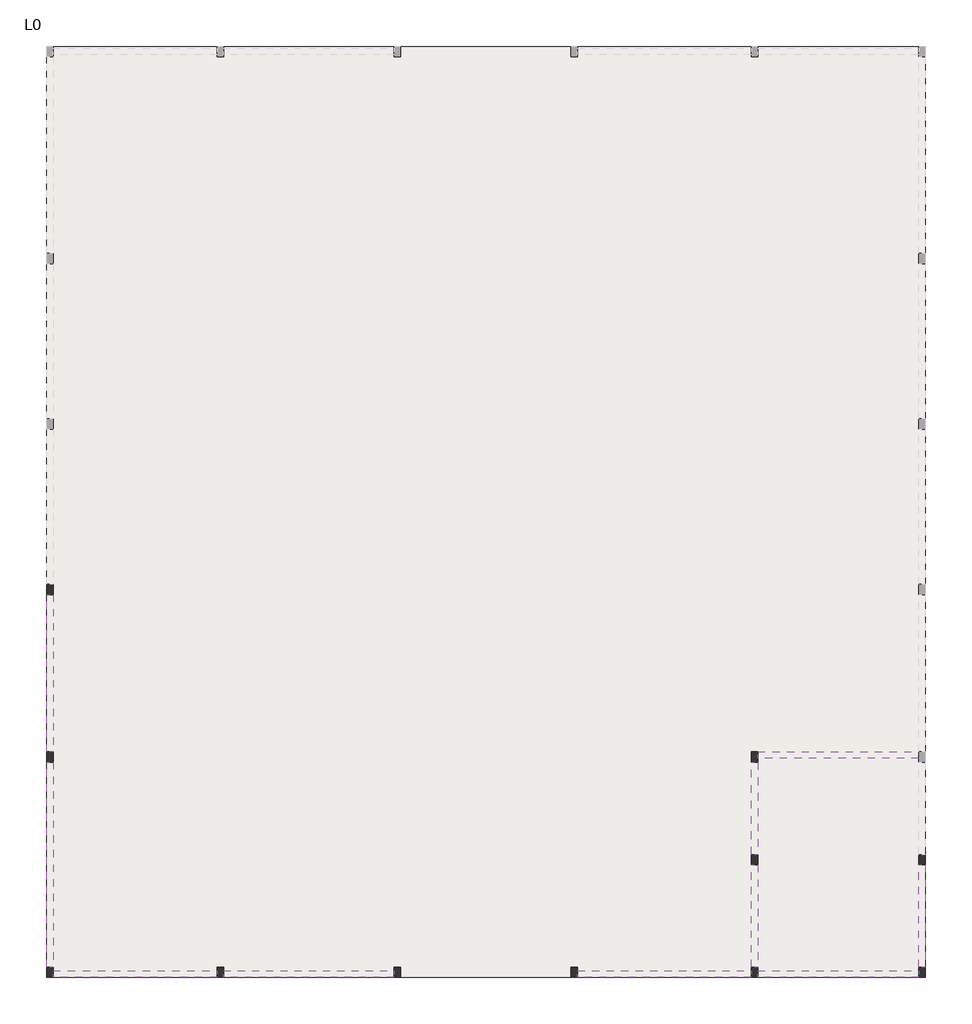
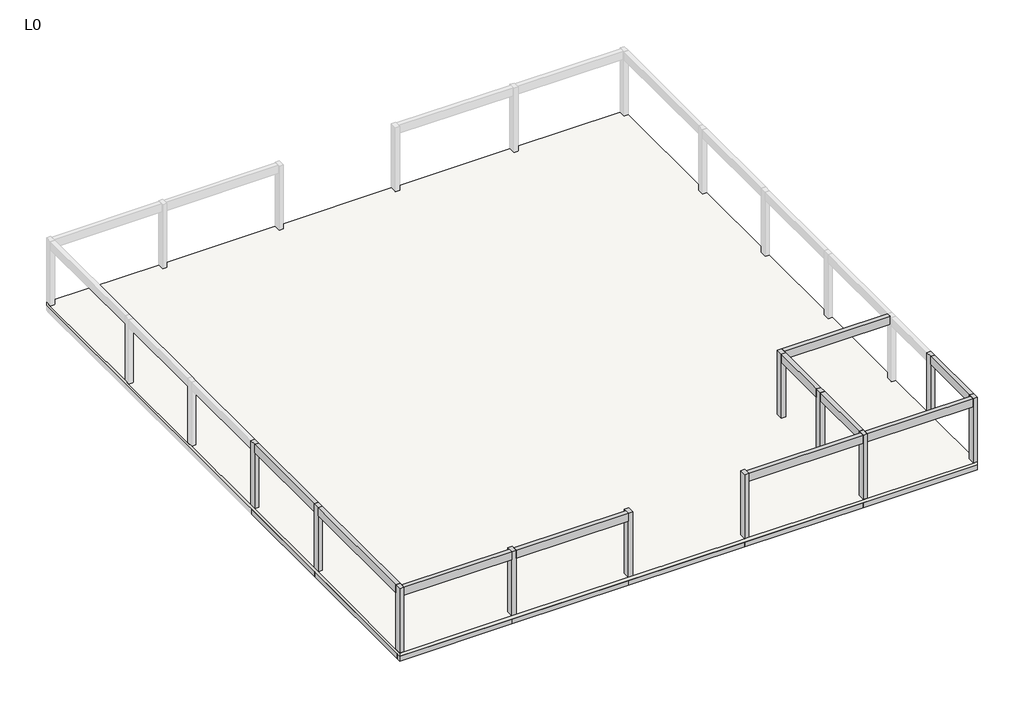
# One storey, part 1 of 2: 32 beams, 11 columns, 1 slab.
"""IFC4 building model written with IfcOpenShell, lengths in millimetres."""

from ifc_helpers import new_model, si_unit, frame, origin, origin_with_axes, place, context, project, spatial, polyline, outline, extrude, faceted_brep, element, save

model = new_model("IFC4")

# Units and contexts
model_context = context("Model", 3, world=origin())
ifc_project = project(units=[si_unit("LENGTHUNIT", "METRE", prefix="MILLI")], contexts=[model_context])

# Site, building, storey
site = spatial("IfcSite", under=ifc_project)
building = spatial("IfcBuilding", under=site)
storey = spatial("IfcBuildingStorey", under=building, Name="L0", Elevation=0.0)

# Beams
placement = place(None, origin())
element("IfcBeam", 1, ObjectType="Concrete-Rectangular Beam : 25 x 50", at=placement, inside=storey, context=model_context, shape_type="Brep", body=[
    faceted_brep([(17000.0, -2875.0, -500.0), (16750.0, -2875.0, -500.0), (10520.0, -2875.0, -500.0), (10520.0, -2875.0, -200.0), (16750.0, -2875.0, -200.0), (17000.0, -2875.0, -200.0), (17000.0, -3125.0, -500.0), (16750.0, -3125.0, -500.0), (10520.0, -3125.0, -500.0), (17000.0, -3125.0, -200.0), (16750.0, -3125.0, -200.0), (10520.0, -3125.0, -200.0)], [[[0, 1, 2, 3, 4, 5]], [[0, 6, 7, 8, 2, 1]], [[8, 7, 6, 9, 10, 11]], [[6, 0, 5, 9]], [[2, 8, 11, 3]], [[5, 4, 3, 11, 10, 9]]]),
])
element("IfcBeam", 2, ObjectType="Concrete-Rectangular Beam : 25 x 50", at=placement, inside=storey, context=model_context, shape_type="Brep", body=[
    faceted_brep([(17000.0, -9345.0, -500.0), (16750.0, -9345.0, -500.0), (10520.0, -9345.0, -500.0), (10270.0, -9345.0, -500.0), (10270.0, -9345.0, -200.0), (10520.0, -9345.0, -200.0), (16750.0, -9345.0, -200.0), (17000.0, -9345.0, -200.0), (10270.0, -9595.0, -500.0), (17000.0, -9595.0, -500.0), (16750.0, -9595.0, -500.0), (10520.0, -9595.0, -500.0), (17000.0, -9595.0, -200.0), (16750.0, -9595.0, -200.0), (10520.0, -9595.0, -200.0), (10270.0, -9595.0, -200.0)], [[[0, 1, 2, 3, 4, 5, 6, 7]], [[8, 3, 2, 1, 0, 9, 10, 11]], [[8, 11, 10, 9, 12, 13, 14, 15]], [[3, 8, 15, 4]], [[9, 0, 7, 12]], [[7, 6, 5, 4, 15, 14, 13, 12]]]),
])
element("IfcBeam", 3, ObjectType="Concrete-Rectangular Beam : 25 x 50", at=placement, inside=storey, context=model_context, shape_type="Brep", body=[
    faceted_brep([(10270.0, -9345.0, -500.0), (3550.0, -9345.0, -500.0), (3300.0, -9345.0, -500.0), (-3300.0, -9345.0, -500.0), (-3300.0, -9345.0, -200.0), (3300.0, -9345.0, -200.0), (3550.0, -9345.0, -200.0), (10270.0, -9345.0, -200.0), (10270.0, -9595.0, -500.0), (3550.0, -9595.0, -500.0), (3300.0, -9595.0, -500.0), (-3300.0, -9595.0, -500.0), (10270.0, -9595.0, -200.0), (3550.0, -9595.0, -200.0), (3300.0, -9595.0, -200.0), (-3300.0, -9595.0, -200.0)], [[[0, 1, 2, 3, 4, 5, 6, 7]], [[0, 8, 9, 10, 11, 3, 2, 1]], [[11, 10, 9, 8, 12, 13, 14, 15]], [[8, 0, 7, 12]], [[3, 11, 15, 4]], [[7, 6, 5, 4, 15, 14, 13, 12]]]),
])
element("IfcBeam", 4, ObjectType="Concrete-Rectangular Beam : 25 x 50", at=placement, inside=storey, context=model_context, shape_type="Brep", body=[
    faceted_brep([(17000.0, -17750.0, -500.0), (16750.0, -17750.0, -500.0), (10520.0, -17750.0, -500.0), (10270.0, -17750.0, -500.0), (10270.0, -17750.0, -200.0), (10520.0, -17750.0, -200.0), (16750.0, -17750.0, -200.0), (17000.0, -17750.0, -200.0), (10270.0, -18000.0, -500.0), (17000.0, -18000.0, -500.0), (17000.0, -18000.0, -200.0), (10270.0, -18000.0, -200.0)], [[[0, 1, 2, 3, 4, 5, 6, 7]], [[8, 3, 2, 1, 0, 9]], [[8, 9, 10, 11]], [[3, 8, 11, 4]], [[9, 0, 7, 10]], [[7, 6, 5, 4, 11, 10]]]),
])
element("IfcBeam", 5, ObjectType="Concrete-Rectangular Beam : 25 x 50", at=placement, inside=storey, context=model_context, shape_type="Brep", body=[
    faceted_brep([(10270.0, -17750.0, -500.0), (3550.0, -17750.0, -500.0), (3300.0, -17750.0, -500.0), (3300.0, -17750.0, -200.0), (3550.0, -17750.0, -200.0), (10270.0, -17750.0, -200.0), (3300.0, -18000.0, -500.0), (10270.0, -18000.0, -500.0), (10270.0, -18000.0, -200.0), (3300.0, -18000.0, -200.0)], [[[0, 1, 2, 3, 4, 5]], [[6, 2, 1, 0, 7]], [[6, 7, 8, 9]], [[2, 6, 9, 3]], [[7, 0, 5, 8]], [[5, 4, 3, 9, 8]]]),
])
element("IfcBeam", 6, ObjectType="Concrete-Rectangular Beam : 25 x 50", at=placement, inside=storey, context=model_context, shape_type="Brep", body=[
    faceted_brep([(3300.0, -17750.0, -500.0), (-3300.0, -17750.0, -500.0), (-3550.0, -17750.0, -500.0), (-3550.0, -17750.0, -200.0), (-3300.0, -17750.0, -200.0), (3300.0, -17750.0, -200.0), (-3550.0, -18000.0, -500.0), (3300.0, -18000.0, -500.0), (3300.0, -18000.0, -200.0), (-3550.0, -18000.0, -200.0)], [[[0, 1, 2, 3, 4, 5]], [[6, 2, 1, 0, 7]], [[6, 7, 8, 9]], [[2, 6, 9, 3]], [[7, 0, 5, 8]], [[5, 4, 3, 9, 8]]]),
])
element("IfcBeam", 7, ObjectType="Concrete-Rectangular Beam : 25 x 50", at=placement, inside=storey, context=model_context, shape_type="Brep", body=[
    faceted_brep([(-3550.0, -17750.0, -500.0), (-10150.0, -17750.0, -500.0), (-10400.0, -17750.0, -500.0), (-10400.0, -17750.0, -200.0), (-10150.0, -17750.0, -200.0), (-3550.0, -17750.0, -200.0), (-10400.0, -18000.0, -500.0), (-3550.0, -18000.0, -500.0), (-3550.0, -18000.0, -200.0), (-10400.0, -18000.0, -200.0)], [[[0, 1, 2, 3, 4, 5]], [[6, 2, 1, 0, 7]], [[6, 7, 8, 9]], [[2, 6, 9, 3]], [[7, 0, 5, 8]], [[5, 4, 3, 9, 8]]]),
])
element("IfcBeam", 8, ObjectType="Concrete-Rectangular Beam : 25 x 50", at=placement, inside=storey, context=model_context, shape_type="Brep", body=[
    faceted_brep([(-10400.0, -17750.0, -500.0), (-16750.0, -17750.0, -500.0), (-17000.0, -17750.0, -500.0), (-17000.0, -17750.0, -200.0), (-16750.0, -17750.0, -200.0), (-10400.0, -17750.0, -200.0), (-10400.0, -18000.0, -500.0), (-17000.0, -18000.0, -500.0), (-10400.0, -18000.0, -200.0), (-17000.0, -18000.0, -200.0)], [[[0, 1, 2, 3, 4, 5]], [[0, 6, 7, 2, 1]], [[7, 6, 8, 9]], [[6, 0, 5, 8]], [[2, 7, 9, 3]], [[5, 4, 3, 9, 8]]]),
])
element("IfcBeam", 9, ObjectType="Concrete-Rectangular Beam : 25 x 50", at=placement, inside=storey, context=model_context, shape_type="Brep", body=[
    faceted_brep([(-16750.0, -17750.0, -500.0), (-16750.0, -9595.0, -500.0), (-16750.0, -9345.0, -500.0), (-16750.0, -9345.0, -200.0), (-16750.0, -9595.0, -200.0), (-16750.0, -17750.0, -200.0), (-17000.0, -9345.0, -500.0), (-17000.0, -17750.0, -500.0), (-17000.0, -17750.0, -200.0), (-17000.0, -9345.0, -200.0)], [[[0, 1, 2, 3, 4, 5]], [[6, 2, 1, 0, 7]], [[6, 7, 8, 9]], [[2, 6, 9, 3]], [[7, 0, 5, 8]], [[5, 4, 3, 9, 8]]]),
])
element("IfcBeam", 10, ObjectType="Concrete-Rectangular Beam : 25 x 50", at=placement, inside=storey, context=model_context, shape_type="Brep", body=[
    faceted_brep([(-16750.0, -9345.0, -500.0), (-16750.0, -3125.0, -500.0), (-16750.0, -2875.0, -500.0), (-16750.0, -2875.0, -200.0), (-16750.0, -3125.0, -200.0), (-16750.0, -9345.0, -200.0), (-17000.0, -2875.0, -500.0), (-17000.0, -9345.0, -500.0), (-17000.0, -9345.0, -200.0), (-17000.0, -2875.0, -200.0)], [[[0, 1, 2, 3, 4, 5]], [[6, 2, 1, 0, 7]], [[6, 7, 8, 9]], [[2, 6, 9, 3]], [[7, 0, 5, 8]], [[5, 4, 3, 9, 8]]]),
])
element("IfcBeam", 11, ObjectType="Concrete-Rectangular Beam : 25 x 50", at=placement, inside=storey, context=model_context, shape_type="SweptSolid", body=[
    extrude(outline(polyline([(-10150.0, -17750.0), (-10400.0, -17750.0), (-10400.0, -9595.0), (-10150.0, -9595.0), (-10150.0, -17750.0)])), frame((0.0, 0.0, -500.0), z_axis=(0.0, 0.0, 1.0), x_axis=(1.0, 0.0, 0.0)), (0.0, 0.0, 1.0), 300.0),
])
element("IfcBeam", 12, ObjectType="Concrete-Rectangular Beam : 25 x 50", at=placement, inside=storey, context=model_context, shape_type="Brep", body=[
    faceted_brep([(-3300.0, -17750.0, -500.0), (-3300.0, -9595.0, -500.0), (-3300.0, -9345.0, -500.0), (-3300.0, -3125.0, -500.0), (-3300.0, -2875.0, -500.0), (-3300.0, 3275.0, -500.0), (-3300.0, 3275.0, -200.0), (-3300.0, -2875.0, -200.0), (-3300.0, -3125.0, -200.0), (-3300.0, -9345.0, -200.0), (-3300.0, -9595.0, -200.0), (-3300.0, -17750.0, -200.0), (-3550.0, -17750.0, -500.0), (-3550.0, -9595.0, -500.0), (-3550.0, -9345.0, -500.0), (-3550.0, -3125.0, -500.0), (-3550.0, -2875.0, -500.0), (-3550.0, 3275.0, -500.0), (-3550.0, -17750.0, -200.0), (-3550.0, -9595.0, -200.0), (-3550.0, -9345.0, -200.0), (-3550.0, -3125.0, -200.0), (-3550.0, -2875.0, -200.0), (-3550.0, 3275.0, -200.0)], [[[0, 1, 2, 3, 4, 5, 6, 7, 8, 9, 10, 11]], [[0, 12, 13, 14, 15, 16, 17, 5, 4, 3, 2, 1]], [[17, 16, 15, 14, 13, 12, 18, 19, 20, 21, 22, 23]], [[12, 0, 11, 18]], [[5, 17, 23, 6]], [[11, 10, 9, 8, 7, 6, 23, 22, 21, 20, 19, 18]]]),
])
element("IfcBeam", 13, ObjectType="Concrete-Rectangular Beam : 25 x 50", at=placement, inside=storey, context=model_context, shape_type="SweptSolid", body=[
    extrude(outline(polyline([(3550.0, -17750.0), (3300.0, -17750.0), (3300.0, -9595.0), (3550.0, -9595.0), (3550.0, -17750.0)])), frame((0.0, 0.0, -500.0), z_axis=(0.0, 0.0, 1.0), x_axis=(1.0, 0.0, 0.0)), (0.0, 0.0, 1.0), 300.0),
])
element("IfcBeam", 14, ObjectType="Concrete-Rectangular Beam : 25 x 50", at=placement, inside=storey, context=model_context, shape_type="SweptSolid", body=[
    extrude(outline(polyline([(10270.0, -13448.5675387), (10520.0, -13448.5675387), (10520.0, -17750.0), (10270.0, -17750.0), (10270.0, -13448.5675387)])), frame((0.0, 0.0, -500.0), z_axis=(0.0, 0.0, 1.0), x_axis=(1.0, 0.0, 0.0)), (0.0, 0.0, 1.0), 300.0),
])
element("IfcBeam", 15, ObjectType="Concrete-Rectangular Beam : 25 x 50", at=placement, inside=storey, context=model_context, shape_type="SweptSolid", body=[
    extrude(outline(polyline([(10520.0, -9595.0), (10520.0, -13448.5675387), (10270.0, -13448.5675387), (10270.0, -9595.0), (10520.0, -9595.0)])), frame((0.0, 0.0, -500.0), z_axis=(0.0, 0.0, 1.0), x_axis=(1.0, 0.0, 0.0)), (0.0, 0.0, 1.0), 300.0),
])
element("IfcBeam", 16, ObjectType="Concrete-Rectangular Beam : 25 x 50", at=placement, inside=storey, context=model_context, shape_type="Brep", body=[
    faceted_brep([(10520.0, -9345.0, -500.0), (10520.0, -3125.0, -500.0), (10520.0, -2875.0, -500.0), (10520.0, 3275.0, -500.0), (10520.0, 3275.0, -200.0), (10520.0, -2875.0, -200.0), (10520.0, -3125.0, -200.0), (10520.0, -9345.0, -200.0), (10270.0, -9345.0, -500.0), (10270.0, -3125.0, -500.0), (10270.0, -2875.0, -500.0), (10270.0, 3275.0, -500.0), (10270.0, -9345.0, -200.0), (10270.0, -3125.0, -200.0), (10270.0, -2875.0, -200.0), (10270.0, 3275.0, -200.0)], [[[0, 1, 2, 3, 4, 5, 6, 7]], [[0, 8, 9, 10, 11, 3, 2, 1]], [[11, 10, 9, 8, 12, 13, 14, 15]], [[8, 0, 7, 12]], [[3, 11, 15, 4]], [[7, 6, 5, 4, 15, 14, 13, 12]]]),
])
element("IfcBeam", 17, ObjectType="Concrete-Rectangular Beam : 25 x 50", at=placement, inside=storey, context=model_context, shape_type="SweptSolid", body=[
    extrude(outline(polyline([(16750.0, -13448.5675387), (17000.0, -13448.5675387), (17000.0, -17750.0), (16750.0, -17750.0), (16750.0, -13448.5675387)])), frame((0.0, 0.0, -500.0), z_axis=(0.0, 0.0, 1.0), x_axis=(1.0, 0.0, 0.0)), (0.0, 0.0, 1.0), 300.0),
])
element("IfcBeam", 18, ObjectType="Concrete-Rectangular Beam : 25 x 50", at=placement, inside=storey, context=model_context, shape_type="SweptSolid", body=[
    extrude(outline(polyline([(-16750.0, -3125.0), (-16750.0, -2875.0), (-10400.0, -2875.0), (-10400.0, -3125.0), (-16750.0, -3125.0)])), frame((0.0, 0.0, -500.0), z_axis=(0.0, 0.0, 1.0), x_axis=(1.0, 0.0, 0.0)), (0.0, 0.0, 1.0), 300.0),
])
element("IfcBeam", 19, ObjectType="Concrete-Rectangular Beam : 25 x 50", at=placement, inside=storey, context=model_context, shape_type="SweptSolid", body=[
    extrude(outline(polyline([(-10150.0, -3125.0), (-10150.0, -2875.0), (-3550.0, -2875.0), (-3550.0, -3125.0), (-10150.0, -3125.0)])), frame((0.0, 0.0, -500.0), z_axis=(0.0, 0.0, 1.0), x_axis=(1.0, 0.0, 0.0)), (0.0, 0.0, 1.0), 300.0),
])
element("IfcBeam", 20, ObjectType="Concrete-Rectangular Beam : 25 x 50", at=placement, inside=storey, context=model_context, shape_type="Brep", body=[
    faceted_brep([(10270.0, -2875.0, -500.0), (3550.0, -2875.0, -500.0), (3300.0, -2875.0, -500.0), (-3300.0, -2875.0, -500.0), (-3300.0, -2875.0, -200.0), (3300.0, -2875.0, -200.0), (3550.0, -2875.0, -200.0), (10270.0, -2875.0, -200.0), (-3300.0, -3125.0, -500.0), (10270.0, -3125.0, -500.0), (3550.0, -3125.0, -500.0), (3300.0, -3125.0, -500.0), (10270.0, -3125.0, -200.0), (3550.0, -3125.0, -200.0), (3300.0, -3125.0, -200.0), (-3300.0, -3125.0, -200.0)], [[[0, 1, 2, 3, 4, 5, 6, 7]], [[8, 3, 2, 1, 0, 9, 10, 11]], [[8, 11, 10, 9, 12, 13, 14, 15]], [[3, 8, 15, 4]], [[9, 0, 7, 12]], [[7, 6, 5, 4, 15, 14, 13, 12]]]),
])
element("IfcBeam", 21, ObjectType="Concrete-Rectangular Beam : 25 x 50", at=placement, inside=storey, context=model_context, shape_type="Brep", body=[
    faceted_brep([(-3550.0, -9345.0, -500.0), (-10150.0, -9345.0, -500.0), (-10400.0, -9345.0, -500.0), (-16750.0, -9345.0, -500.0), (-16750.0, -9345.0, -200.0), (-10400.0, -9345.0, -200.0), (-10150.0, -9345.0, -200.0), (-3550.0, -9345.0, -200.0), (-16750.0, -9595.0, -500.0), (-3550.0, -9595.0, -500.0), (-10150.0, -9595.0, -500.0), (-10400.0, -9595.0, -500.0), (-3550.0, -9595.0, -200.0), (-10150.0, -9595.0, -200.0), (-10400.0, -9595.0, -200.0), (-16750.0, -9595.0, -200.0)], [[[0, 1, 2, 3, 4, 5, 6, 7]], [[8, 3, 2, 1, 0, 9, 10, 11]], [[8, 11, 10, 9, 12, 13, 14, 15]], [[3, 8, 15, 4]], [[9, 0, 7, 12]], [[7, 6, 5, 4, 15, 14, 13, 12]]]),
])
element("IfcBeam", 22, ObjectType="Concrete-Rectangular Beam : 25 x 50", at=placement, inside=storey, context=model_context, shape_type="SweptSolid", body=[
    extrude(outline(polyline([(3300.0, -3125.0), (3550.0, -3125.0), (3550.0, -9345.0), (3300.0, -9345.0), (3300.0, -3125.0)])), frame((0.0, 0.0, -500.0), z_axis=(0.0, 0.0, 1.0), x_axis=(1.0, 0.0, 0.0)), (0.0, 0.0, 1.0), 300.0),
])
element("IfcBeam", 23, ObjectType="Concrete-Rectangular Beam : 25 x 50", at=placement, inside=storey, context=model_context, shape_type="SweptSolid", body=[
    extrude(outline(polyline([(16750.0, -9270.0), (16750.0, -9520.0), (10520.0, -9520.0), (10520.0, -9270.0), (16750.0, -9270.0)])), frame((0.0, 0.0, 3500.0), z_axis=(0.0, 0.0, 1.0), x_axis=(1.0, 0.0, 0.0)), (0.0, 0.0, 1.0), 500.0),
])
element("IfcBeam", 24, ObjectType="Concrete-Rectangular Beam : 25 x 50", at=placement, inside=storey, context=model_context, shape_type="SweptSolid", body=[
    extrude(outline(polyline([(10520.0, -18000.0), (10520.0, -17750.0), (16750.0, -17750.0), (16750.0, -18000.0), (10520.0, -18000.0)])), frame((0.0, 0.0, 3500.0), z_axis=(0.0, 0.0, 1.0), x_axis=(1.0, 0.0, 0.0)), (0.0, 0.0, 1.0), 500.0),
])
element("IfcBeam", 25, ObjectType="Concrete-Rectangular Beam : 25 x 50", at=placement, inside=storey, context=model_context, shape_type="SweptSolid", body=[
    extrude(outline(polyline([(3550.0, -18000.0), (3550.0, -17750.0), (10270.0, -17750.0), (10270.0, -18000.0), (3550.0, -18000.0)])), frame((0.0, 0.0, 3500.0), z_axis=(0.0, 0.0, 1.0), x_axis=(1.0, 0.0, 0.0)), (0.0, 0.0, 1.0), 500.0),
])
element("IfcBeam", 26, ObjectType="Concrete-Rectangular Beam : 25 x 50", at=placement, inside=storey, context=model_context, shape_type="SweptSolid", body=[
    extrude(outline(polyline([(-10150.0, -18000.0), (-10150.0, -17750.0), (-3550.0, -17750.0), (-3550.0, -18000.0), (-10150.0, -18000.0)])), frame((0.0, 0.0, 3500.0), z_axis=(0.0, 0.0, 1.0), x_axis=(1.0, 0.0, 0.0)), (0.0, 0.0, 1.0), 500.0),
])
element("IfcBeam", 27, ObjectType="Concrete-Rectangular Beam : 25 x 50", at=placement, inside=storey, context=model_context, shape_type="SweptSolid", body=[
    extrude(outline(polyline([(-16750.0, -18000.0), (-16750.0, -17750.0), (-10400.0, -17750.0), (-10400.0, -18000.0), (-16750.0, -18000.0)])), frame((0.0, 0.0, 3500.0), z_axis=(0.0, 0.0, 1.0), x_axis=(1.0, 0.0, 0.0)), (0.0, 0.0, 1.0), 500.0),
])
element("IfcBeam", 28, ObjectType="Concrete-Rectangular Beam : 25 x 50", at=placement, inside=storey, context=model_context, shape_type="SweptSolid", body=[
    extrude(outline(polyline([(-17000.0, -9670.0), (-16750.0, -9670.0), (-16750.0, -17600.0), (-17000.0, -17600.0), (-17000.0, -9670.0)])), frame((0.0, 0.0, 3500.0), z_axis=(0.0, 0.0, 1.0), x_axis=(1.0, 0.0, 0.0)), (0.0, 0.0, 1.0), 500.0),
])
element("IfcBeam", 29, ObjectType="Concrete-Rectangular Beam : 25 x 50", at=placement, inside=storey, context=model_context, shape_type="SweptSolid", body=[
    extrude(outline(polyline([(-17000.0, -3200.0), (-16750.0, -3200.0), (-16750.0, -9270.0), (-17000.0, -9270.0), (-17000.0, -3200.0)])), frame((0.0, 0.0, 3500.0), z_axis=(0.0, 0.0, 1.0), x_axis=(1.0, 0.0, 0.0)), (0.0, 0.0, 1.0), 500.0),
])
element("IfcBeam", 30, ObjectType="Concrete-Rectangular Beam : 25 x 50", at=placement, inside=storey, context=model_context, shape_type="SweptSolid", body=[
    extrude(outline(polyline([(10520.0, -17600.0), (10270.0, -17600.0), (10270.0, -13648.5675387), (10520.0, -13648.5675387), (10520.0, -17600.0)])), frame((0.0, 0.0, 3500.0), z_axis=(0.0, 0.0, 1.0), x_axis=(1.0, 0.0, 0.0)), (0.0, 0.0, 1.0), 500.0),
])
element("IfcBeam", 31, ObjectType="Concrete-Rectangular Beam : 25 x 50", at=placement, inside=storey, context=model_context, shape_type="SweptSolid", body=[
    extrude(outline(polyline([(10520.0, -13248.5675387), (10270.0, -13248.5675387), (10270.0, -9670.0), (10520.0, -9670.0), (10520.0, -13248.5675387)])), frame((0.0, 0.0, 3500.0), z_axis=(0.0, 0.0, 1.0), x_axis=(1.0, 0.0, 0.0)), (0.0, 0.0, 1.0), 500.0),
])
element("IfcBeam", 32, ObjectType="Concrete-Rectangular Beam : 25 x 50", at=placement, inside=storey, context=model_context, shape_type="SweptSolid", body=[
    extrude(outline(polyline([(17000.0, -17600.0), (16750.0, -17600.0), (16750.0, -13648.5675387), (17000.0, -13648.5675387), (17000.0, -17600.0)])), frame((0.0, 0.0, 3500.0), z_axis=(0.0, 0.0, 1.0), x_axis=(1.0, 0.0, 0.0)), (0.0, 0.0, 1.0), 500.0),
])

# Columns
element("IfcColumn", 33, ObjectType="M_Concrete-Rectangular-Column : 250 x 400mm", at=placement, inside=storey, context=model_context, shape_type="SweptSolid", body=[
    extrude(outline(polyline([(-17000.0, -3200.0), (-17000.0, -2800.0), (-16750.0, -2800.0), (-16750.0, -3200.0), (-17000.0, -3200.0)])), origin_with_axes(), (0.0, 0.0, 1.0), 4000.0),
])
element("IfcColumn", 34, ObjectType="M_Concrete-Rectangular-Column : 250 x 400mm", at=placement, inside=storey, context=model_context, shape_type="SweptSolid", body=[
    extrude(outline(polyline([(-17000.0, -9670.0), (-17000.0, -9270.0), (-16750.0, -9270.0), (-16750.0, -9670.0), (-17000.0, -9670.0)])), origin_with_axes(), (0.0, 0.0, 1.0), 4000.0),
])
element("IfcColumn", 35, ObjectType="M_Concrete-Rectangular-Column : 250 x 400mm", at=placement, inside=storey, context=model_context, shape_type="SweptSolid", body=[
    extrude(outline(polyline([(-17000.0, -18000.0), (-17000.0, -17600.0), (-16750.0, -17600.0), (-16750.0, -18000.0), (-17000.0, -18000.0)])), origin_with_axes(), (0.0, 0.0, 1.0), 4000.0),
])
element("IfcColumn", 36, ObjectType="M_Concrete-Rectangular-Column : 250 x 400mm", at=placement, inside=storey, context=model_context, shape_type="SweptSolid", body=[
    extrude(outline(polyline([(-10400.0, -18000.0), (-10400.0, -17600.0), (-10150.0, -17600.0), (-10150.0, -18000.0), (-10400.0, -18000.0)])), origin_with_axes(), (0.0, 0.0, 1.0), 4000.0),
])
element("IfcColumn", 37, ObjectType="M_Concrete-Rectangular-Column : 250 x 400mm", at=placement, inside=storey, context=model_context, shape_type="SweptSolid", body=[
    extrude(outline(polyline([(-3550.0, -18000.0), (-3550.0, -17600.0), (-3300.0, -17600.0), (-3300.0, -18000.0), (-3550.0, -18000.0)])), origin_with_axes(), (0.0, 0.0, 1.0), 4000.0),
])
element("IfcColumn", 38, ObjectType="M_Concrete-Rectangular-Column : 250 x 400mm", at=placement, inside=storey, context=model_context, shape_type="SweptSolid", body=[
    extrude(outline(polyline([(3300.0, -18000.0), (3300.0, -17600.0), (3550.0, -17600.0), (3550.0, -18000.0), (3300.0, -18000.0)])), origin_with_axes(), (0.0, 0.0, 1.0), 4000.0),
])
element("IfcColumn", 39, ObjectType="M_Concrete-Rectangular-Column : 250 x 400mm", at=placement, inside=storey, context=model_context, shape_type="SweptSolid", body=[
    extrude(outline(polyline([(10270.0, -18000.0), (10270.0, -17600.0), (10520.0, -17600.0), (10520.0, -18000.0), (10270.0, -18000.0)])), origin_with_axes(), (0.0, 0.0, 1.0), 4000.0),
])
element("IfcColumn", 40, ObjectType="M_Concrete-Rectangular-Column : 250 x 400mm", at=placement, inside=storey, context=model_context, shape_type="SweptSolid", body=[
    extrude(outline(polyline([(17000.0, -17600.0), (17000.0, -18000.0), (16750.0, -18000.0), (16750.0, -17600.0), (17000.0, -17600.0)])), origin_with_axes(), (0.0, 0.0, 1.0), 4000.0),
])
element("IfcColumn", 41, ObjectType="M_Concrete-Rectangular-Column : 250 x 400mm", at=placement, inside=storey, context=model_context, shape_type="SweptSolid", body=[
    extrude(outline(polyline([(10520.0, -13248.5675387), (10520.0, -13648.5675387), (10270.0, -13648.5675387), (10270.0, -13248.5675387), (10520.0, -13248.5675387)])), origin_with_axes(), (0.0, 0.0, 1.0), 4000.0),
])
element("IfcColumn", 42, ObjectType="M_Concrete-Rectangular-Column : 250 x 400mm", at=placement, inside=storey, context=model_context, shape_type="SweptSolid", body=[
    extrude(outline(polyline([(17000.0, -13248.5675387), (17000.0, -13648.5675387), (16750.0, -13648.5675387), (16750.0, -13248.5675387), (17000.0, -13248.5675387)])), origin_with_axes(), (0.0, 0.0, 1.0), 4000.0),
])
element("IfcColumn", 43, ObjectType="M_Concrete-Rectangular-Column : 250 x 400mm", at=placement, inside=storey, context=model_context, shape_type="SweptSolid", body=[
    extrude(outline(polyline([(10520.0, -9270.0), (10520.0, -9670.0), (10270.0, -9670.0), (10270.0, -9270.0), (10520.0, -9270.0)])), origin_with_axes(), (0.0, 0.0, 1.0), 4000.0),
])

# Slab
element("IfcSlab", 44, ObjectType="Generic 200mm DAPC", at=placement, inside=storey, context=model_context, shape_type="Brep", body=[
    faceted_brep([(17000.0, 18000.0, -200.0), (17000.0, 17750.0, -200.0), (17000.0, 9925.0, -200.0), (17000.0, 9675.0, -200.0), (17000.0, 3525.0, -200.0), (17000.0, 3275.0, -200.0), (17000.0, -2875.0, -200.0), (17000.0, -3125.0, -200.0), (17000.0, -9345.0, -200.0), (17000.0, -9595.0, -200.0), (17000.0, -13448.5675387, -200.0), (17000.0, -17750.0, -200.0), (17000.0, -18000.0, -200.0), (10270.0, -18000.0, -200.0), (3300.0, -18000.0, -200.0), (-3550.0, -18000.0, -200.0), (-10400.0, -18000.0, -200.0), (-17000.0, -18000.0, -200.0), (-17000.0, -17750.0, -200.0), (-17000.0, -9345.0, -200.0), (-17000.0, -2875.0, -200.0), (-17000.0, 3525.0, -200.0), (-17000.0, 9925.0, -200.0), (-17000.0, 17750.0, -200.0), (-17000.0, 18000.0, -200.0), (-10400.0, 18000.0, -200.0), (-3550.0, 18000.0, -200.0), (3300.0, 18000.0, -200.0), (10270.0, 18000.0, -200.0), (17000.0, 18000.0, 0.0), (16750.0, 18000.0, 0.0), (10520.0, 18000.0, 0.0), (10270.0, 18000.0, 0.0), (3550.0, 18000.0, 0.0), (3300.0, 18000.0, 0.0), (-3300.0, 18000.0, 0.0), (-3550.0, 18000.0, 0.0), (-10150.0, 18000.0, 0.0), (-10400.0, 18000.0, 0.0), (-16750.0, 18000.0, 0.0), (-17000.0, 18000.0, 0.0), (-17000.0, 17600.0, 0.0), (-17000.0, 10000.0, 0.0), (-17000.0, 9600.0, 0.0), (-17000.0, 3600.0, 0.0), (-17000.0, 3200.0, 0.0), (-17000.0, -2800.0, 0.0), (-17000.0, -3200.0, 0.0), (-17000.0, -9270.0, 0.0), (-17000.0, -9670.0, 0.0), (-17000.0, -17600.0, 0.0), (-17000.0, -18000.0, 0.0), (-16750.0, -18000.0, 0.0), (-10400.0, -18000.0, 0.0), (-10150.0, -18000.0, 0.0), (-3550.0, -18000.0, 0.0), (-3300.0, -18000.0, 0.0), (3300.0, -18000.0, 0.0), (3550.0, -18000.0, 0.0), (10270.0, -18000.0, 0.0), (10520.0, -18000.0, 0.0), (16750.0, -18000.0, 0.0), (17000.0, -18000.0, 0.0), (17000.0, -17600.0, 0.0), (17000.0, -13648.5675387, 0.0), (17000.0, -13248.5675387, 0.0), (17000.0, -9670.0, 0.0), (17000.0, -9270.0, 0.0), (17000.0, -3200.0, 0.0), (17000.0, -2800.0, 0.0), (17000.0, 3200.0, 0.0), (17000.0, 3600.0, 0.0), (17000.0, 9600.0, 0.0), (17000.0, 10000.0, 0.0), (17000.0, 17600.0, 0.0)], [[[0, 1, 2, 3, 4, 5, 6, 7, 8, 9, 10, 11, 12, 13, 14, 15, 16, 17, 18, 19, 20, 21, 22, 23, 24, 25, 26, 27, 28]], [[29, 30, 31, 32, 33, 34, 35, 36, 37, 38, 39, 40, 41, 42, 43, 44, 45, 46, 47, 48, 49, 50, 51, 52, 53, 54, 55, 56, 57, 58, 59, 60, 61, 62, 63, 64, 65, 66, 67, 68, 69, 70, 71, 72, 73, 74]], [[12, 11, 10, 9, 8, 7, 6, 5, 4, 3, 2, 1, 0, 29, 74, 73, 72, 71, 70, 69, 68, 67, 66, 65, 64, 63, 62]], [[17, 16, 15, 14, 13, 12, 62, 61, 60, 59, 58, 57, 56, 55, 54, 53, 52, 51]], [[24, 23, 22, 21, 20, 19, 18, 17, 51, 50, 49, 48, 47, 46, 45, 44, 43, 42, 41, 40]], [[0, 28, 27, 26, 25, 24, 40, 39, 38, 37, 36, 35, 34, 33, 32, 31, 30, 29]]]),
])

save(model, "model.ifc")

# Revit data of these elements
# Project information
#   Organization Name = "Organization Name"
#   Organization Description = "Organization Description"
#   Building Name = "Building Name"
#   Project Issue Date = "Issue Date"
#   Project Status = "Project Status"
#   Client Name = "Client Name"
#   Project Address = "Enter address here\nAddress Line 2"
#   Project Name = "Project Name"
#   Project Number = "Project Number"
# Grids (mm)
#   "6": line (-18973.453, -17800) -> (19013.601, -17800)
#   "A": line (-16875, 19761.018) -> (-16875, -19399.989)
#   "F": line (16875, 19761.018) -> (16875, -19399.989)
#   "1": line (-18973.453, 17800) -> (19013.601, 17800)
# Type "Concrete-Rectangular Beam : 25 x 50"
#   Length [instance default] = 1.524 m
#   b = 0.25 m
#   h = 0.50 m
#   Structural Material [instance default] = Concrete, Cast-in-Place gray
#   Assembly Code = ""
# Type "M_Concrete-Rectangular-Column : 250 x 400mm"
#   b = 0.25 m
#   h = 0.40 m
#   Structural Material [instance default] = Concrete, Cast-in-Place gray
# Type "Generic 200mm DAPC"
#   Description = "Generic Floor (Material By Category), 300mm thick"
#   Function = 0
#   Layers, outside or top first: 0.20 m "Concrete, Lightweight" (function 1)
# Elements 1, 2, 4, 23, 24 (IfcBeam, "Concrete-Rectangular Beam : 25 x 50")
#   Length = 6.48 m
#   Structural Material = Concrete, Cast-in-Place gray
#   Phase Created = New Construction
#   Materials on its faces: "Concrete, Cast-in-Place gray"
# Element 3 (IfcBeam, "Concrete-Rectangular Beam : 25 x 50")
#   Length = 13.82 m
#   Structural Material = Concrete, Cast-in-Place gray
#   Phase Created = New Construction
#   Materials on its faces: "Concrete, Cast-in-Place gray"
# Elements 5, 25 (IfcBeam, "Concrete-Rectangular Beam : 25 x 50")
#   Length = 6.97 m
#   Structural Material = Concrete, Cast-in-Place gray
#   Phase Created = New Construction
#   Materials on its faces: "Concrete, Cast-in-Place gray"
# Elements 6, 7, 26 (IfcBeam, "Concrete-Rectangular Beam : 25 x 50")
#   Length = 6.85 m
#   Structural Material = Concrete, Cast-in-Place gray
#   Phase Created = New Construction
#   Materials on its faces: "Concrete, Cast-in-Place gray"
# Elements 8, 27 (IfcBeam, "Concrete-Rectangular Beam : 25 x 50")
#   Length = 6.60 m
#   Structural Material = Concrete, Cast-in-Place gray
#   Phase Created = New Construction
#   Materials on its faces: "Concrete, Cast-in-Place gray"
# Elements 9, 11, 13 (IfcBeam, "Concrete-Rectangular Beam : 25 x 50")
#   Length = 8.405 m
#   Structural Material = Concrete, Cast-in-Place gray
#   Phase Created = New Construction
#   Materials on its faces: "Concrete, Cast-in-Place gray"
# Elements 10, 29 (IfcBeam, "Concrete-Rectangular Beam : 25 x 50")
#   Length = 6.47 m
#   Structural Material = Concrete, Cast-in-Place gray
#   Phase Created = New Construction
#   Materials on its faces: "Concrete, Cast-in-Place gray"
# Element 12 (IfcBeam, "Concrete-Rectangular Beam : 25 x 50")
#   Length = 21.275 m
#   Structural Material = Concrete, Cast-in-Place gray
#   Phase Created = New Construction
#   Materials on its faces: "Concrete, Cast-in-Place gray"
# Elements 14, 17 (IfcBeam, "Concrete-Rectangular Beam : 25 x 50")
#   Length = 4.426432 m
#   Structural Material = Concrete, Cast-in-Place gray
#   Phase Created = New Construction
#   Materials on its faces: "Concrete, Cast-in-Place gray"
# Elements 15, 31 (IfcBeam, "Concrete-Rectangular Beam : 25 x 50")
#   Length = 3.978568 m
#   Structural Material = Concrete, Cast-in-Place gray
#   Phase Created = New Construction
#   Materials on its faces: "Concrete, Cast-in-Place gray"
# Element 16 (IfcBeam, "Concrete-Rectangular Beam : 25 x 50")
#   Length = 12.87 m
#   Structural Material = Concrete, Cast-in-Place gray
#   Phase Created = New Construction
#   Materials on its faces: "Concrete, Cast-in-Place gray"
# Elements 18, 19, 20 (IfcBeam, "Concrete-Rectangular Beam : 25 x 50")
#   IfcGUID = "2BzmfI2393bxdTxu7BJEPc"
#   Phase Created = New Construction
#   Materials on its faces: "Concrete, Cast-in-Place gray"
# Element 21 (IfcBeam, "Concrete-Rectangular Beam : 25 x 50")
#   IfcGUID = "2BzmfI2393bxdTxu7BJEPa"
#   Phase Created = New Construction
#   Materials on its faces: "Concrete, Cast-in-Place gray"
# Element 22 (IfcBeam, "Concrete-Rectangular Beam : 25 x 50")
#   IfcGUID = "2BzmfI2393bxdTxu7BJEPx"
#   Phase Created = New Construction
#   Materials on its faces: "Concrete, Cast-in-Place gray"
# Element 28 (IfcBeam, "Concrete-Rectangular Beam : 25 x 50")
#   Length = 8.33 m
#   Structural Material = Concrete, Cast-in-Place gray
#   Phase Created = New Construction
#   Materials on its faces: "Concrete, Cast-in-Place gray"
# Elements 30, 32 (IfcBeam, "Concrete-Rectangular Beam : 25 x 50")
#   Length = 4.351432 m
#   Structural Material = Concrete, Cast-in-Place gray
#   Phase Created = New Construction
#   Materials on its faces: "Concrete, Cast-in-Place gray"
# Elements 33, 34, 35, 36, 37, 38, 39, 40, 41, 42, 43 (IfcColumn, "M_Concrete-Rectangular-Column : 250 x 400mm")
#   Structural Material = Concrete, Cast-in-Place gray
#   Phase Created = New Construction
#   Materials on its faces: "Concrete, Cast-in-Place gray"
# Element 44 (IfcSlab, "Generic 200mm DAPC")
#   Height Offset From Level = 0.00 m
#   built-in parameter 1001954 = 1
#   Phase Created = New Construction
#   Materials on its faces: "Concrete, Lightweight"
# Materials
#   "Concrete, Cast-in-Place gray": class "Concrete", colour RGB 192 192 192, transparency 0, Description = "Cast-in-place concrete", Cost = 0
#   "Concrete, Lightweight": class "Concrete", colour RGB 185 232 147, transparency 0, Description = "Lightweight concrete", Cost = 0
